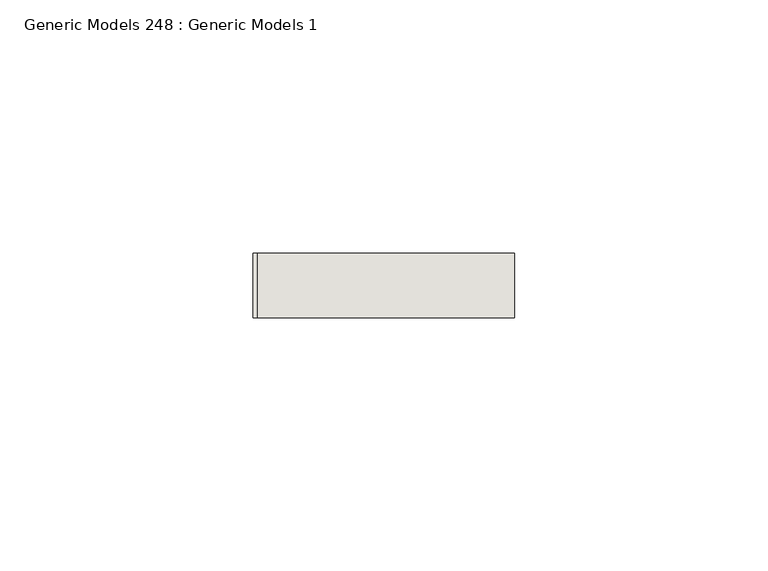
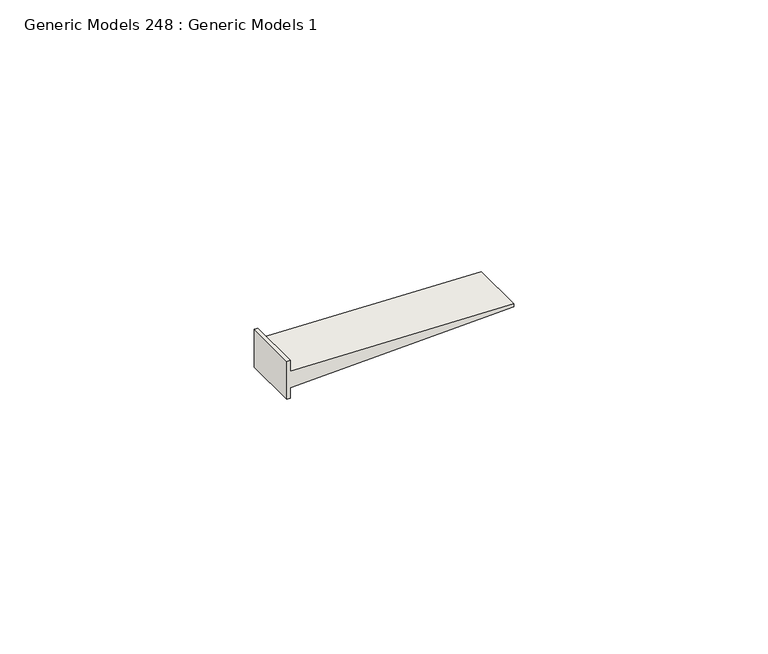
"""IFC4 building model written with IfcOpenShell, lengths in millimetres: wall geometry, Generic Models 248 : Generic Models 1."""

import ifcopenshell
import ifcopenshell.guid

model = None  # the IFC model being written
_history = None  # IfcOwnerHistory: only IFC2X3 demands one
_inside = {}  # id of a spatial element -> (the spatial element, [elements in it])
_under = {}  # id of a project, library or spatial element -> (it, [spatial elements below it])
_declared = {}  # id of a project -> (the project, [libraries it declares])
_typed = {}  # id of a type object -> (the type object, [elements of that type])
_made_of = {}  # id of a material, layer set ... -> (it, [elements and type objects made of it])


def new_model(schema):
    """Start an empty IFC model of exactly this schema.

    Asked for "IFC4X3", IfcOpenShell would pick the latest addendum, in which some entities
    have other attributes; the version numbers below select the first issue.
    IFC2X3 requires an IfcOwnerHistory on every rooted entity: one is made here for all.
    """
    global model, _history
    if schema == "IFC4X3":
        model = ifcopenshell.file(schema_version=(4, 3, 0, 0))
    else:
        model = ifcopenshell.file(schema=schema)
    _inside.clear()
    _under.clear()
    _declared.clear()
    _typed.clear()
    _made_of.clear()
    _history = None
    if model.schema == "IFC2X3":
        org = make("IfcOrganization", Name="unknown")
        user = make(
            "IfcPersonAndOrganization",
            ThePerson=make("IfcPerson", FamilyName="unknown"),
            TheOrganization=org,
        )
        app = make(
            "IfcApplication",
            ApplicationDeveloper=org,
            Version="unknown",
            ApplicationFullName="unknown",
            ApplicationIdentifier="unknown",
        )
        _history = make(
            "IfcOwnerHistory",
            OwningUser=user,
            OwningApplication=app,
            ChangeAction="ADDED",
            CreationDate=0,
        )
    return model


def make(cls, **values):
    """One entity of the class cls with the attributes given. An attribute that is None is left unset."""
    return model.create_entity(
        cls, **{name: value for name, value in values.items() if value is not None}
    )


def rooted(cls, **values):
    """An entity with a GlobalId (a new one), such as an element, a storey or a relation."""
    return make(cls, GlobalId=ifcopenshell.guid.new(), OwnerHistory=_history, **values)


def si_unit(unit_type, name, prefix=None):
    """IfcSIUnit, for example si_unit("LENGTHUNIT", "METRE", prefix="MILLI")."""
    return make("IfcSIUnit", UnitType=unit_type, Prefix=prefix, Name=name)


def assignment(units):
    """IfcUnitAssignment: the units of a project."""
    return None if units is None else make("IfcUnitAssignment", Units=units)


def point(xyz):
    """IfcCartesianPoint."""
    return None if xyz is None else make("IfcCartesianPoint", Coordinates=xyz)


def direction(xyz):
    """IfcDirection."""
    return None if xyz is None else make("IfcDirection", DirectionRatios=xyz)


def frame(location, z_axis=None, x_axis=None):
    """IfcAxis2Placement3D, a coordinate frame: its origin and axes. An axis left out is left unset."""
    return make(
        "IfcAxis2Placement3D",
        Location=point(location),
        Axis=direction(z_axis),
        RefDirection=direction(x_axis),
    )


def origin():
    """The frame at (0, 0, 0) with its axes left unset."""
    return frame((0.0, 0.0, 0.0))


def place(relative_to, where):
    """IfcLocalPlacement: puts the frame where relative to a parent placement (None: the world)."""
    return make(
        "IfcLocalPlacement", PlacementRelTo=relative_to, RelativePlacement=where
    )


def context(
    kind, dimensions, precision=None, world=None, true_north=None, identifier=None
):
    """IfcGeometricRepresentationContext, for example the 3D "Model" context."""
    return make(
        "IfcGeometricRepresentationContext",
        ContextIdentifier=identifier,
        ContextType=kind,
        CoordinateSpaceDimension=dimensions,
        Precision=precision,
        WorldCoordinateSystem=world,
        TrueNorth=true_north,
    )


def project(units=None, contexts=None):
    """IfcProject with its units and contexts."""
    return rooted(
        "IfcProject",
        Name="project",
        RepresentationContexts=contexts,
        UnitsInContext=assignment(units),
    )


def spatial(cls, under=None, at=None, **own):
    """A site, building, storey or space (cls), placed at a placement, below another one or the project."""
    s = rooted(cls, ObjectPlacement=at, **own)
    if under is not None:
        _under.setdefault(under.id(), (under, []))[1].append(s)
    return s


def polyline(points):
    """IfcPolyline through the points."""
    return make("IfcPolyline", Points=[point(p) for p in points])


def outline(outer, holes=None, kind="AREA"):
    """IfcArbitraryClosedProfileDef: a profile drawn as a closed curve; with holes, ...WithVoids."""
    if holes is None:
        return make("IfcArbitraryClosedProfileDef", ProfileType=kind, OuterCurve=outer)
    return make(
        "IfcArbitraryProfileDefWithVoids",
        ProfileType=kind,
        OuterCurve=outer,
        InnerCurves=holes,
    )


def extrude(swept, where, along, depth):
    """IfcExtrudedAreaSolid: the profile swept, set in the frame where, extruded along a direction by depth."""
    return make(
        "IfcExtrudedAreaSolid",
        SweptArea=swept,
        Position=where,
        ExtrudedDirection=direction(along),
        Depth=depth,
    )


def shape(context_of_items, identifier, shape_type, items):
    """IfcShapeRepresentation: the items that make up one representation, for example the "Body"."""
    return make(
        "IfcShapeRepresentation",
        ContextOfItems=context_of_items,
        RepresentationIdentifier=identifier,
        RepresentationType=shape_type,
        Items=items,
    )


def source(mapping_origin, context_of_items, identifier, shape_type, items):
    """IfcRepresentationMap: a shape defined once, which mapped items show again and again."""
    return make(
        "IfcRepresentationMap",
        MappingOrigin=mapping_origin,
        MappedRepresentation=shape(context_of_items, identifier, shape_type, items),
    )


def transform(
    local_origin,
    x_axis=None,
    y_axis=None,
    z_axis=None,
    scale=None,
    scale2=None,
    scale3=None,
    uniform=True,
):
    """IfcCartesianTransformationOperator3D, or its non-uniform kind. x_axis, y_axis, z_axis: its Axis1, 2, 3."""
    if uniform:
        return make(
            "IfcCartesianTransformationOperator3D",
            Axis1=direction(x_axis),
            Axis2=direction(y_axis),
            LocalOrigin=point(local_origin),
            Scale=scale,
            Axis3=direction(z_axis),
        )
    return make(
        "IfcCartesianTransformationOperator3DnonUniform",
        Axis1=direction(x_axis),
        Axis2=direction(y_axis),
        LocalOrigin=point(local_origin),
        Scale=scale,
        Axis3=direction(z_axis),
        Scale2=scale2,
        Scale3=scale3,
    )


def mapped(mapping_source, mapping_target):
    """IfcMappedItem: shows the shape of a source again, moved by a transform."""
    return make(
        "IfcMappedItem", MappingSource=mapping_source, MappingTarget=mapping_target
    )


def made_of(thing, what):
    """Note that an element or type object is made of a material, layer set ...; save() writes the relation."""
    if what is not None:
        _made_of.setdefault(what.id(), (what, []))[1].append(thing)
    return thing


def element(
    cls,
    number,
    at=None,
    inside=None,
    cuts=None,
    type_object=None,
    material=None,
    context=None,
    identifier="Body",
    shape_type=None,
    held_by="IfcProductDefinitionShape",
    body=None,
    shapes=None,
    **own,
):
    """One element of the class cls, such as IfcWall. Its Tag is "e" and its number.

    at: its placement. inside: the storey or other place that contains it. cuts: it is an
    opening in that element (IfcRelVoidsElement). A single representation is given by context,
    identifier, shape_type and body (its items); several are given by shapes. held_by: the class
    of the entity that holds the representations. save() writes the other relations.
    """
    e = rooted(cls, Tag="e%d" % number, ObjectPlacement=at, **own)
    if body is not None:
        shapes = [shape(context, identifier, shape_type, body)]
    if shapes is not None:
        e.Representation = make(held_by, Representations=shapes)
    if inside is not None:
        _inside.setdefault(inside.id(), (inside, []))[1].append(e)
    if cuts is not None:
        rooted(
            "IfcRelVoidsElement", RelatingBuildingElement=cuts, RelatedOpeningElement=e
        )
    if type_object is not None:
        _typed.setdefault(type_object.id(), (type_object, []))[1].append(e)
    return made_of(e, material)


def aggregate(whole, parts):
    """IfcRelAggregates: a whole, such as a stair, and the parts it consists of."""
    return rooted("IfcRelAggregates", RelatingObject=whole, RelatedObjects=parts)


def save(model, path):
    """Write the relations noted so far, then the file.

    IfcRelAggregates (storeys below a building ...), IfcRelContainedInSpatialStructure (elements
    in a storey), IfcRelDefinesByType, IfcRelAssociatesMaterial and IfcRelDeclares: one each for
    every whole, place, type object, material and project.
    """
    for whole, parts in _under.values():
        aggregate(whole, parts)
    for where, things in _inside.values():
        rooted(
            "IfcRelContainedInSpatialStructure",
            RelatedElements=things,
            RelatingStructure=where,
        )
    for kind, things in _typed.values():
        rooted("IfcRelDefinesByType", RelatedObjects=things, RelatingType=kind)
    for what, things in _made_of.values():
        rooted("IfcRelAssociatesMaterial", RelatedObjects=things, RelatingMaterial=what)
    for by, libraries in _declared.values():
        rooted("IfcRelDeclares", RelatingContext=by, RelatedDefinitions=libraries)
    model.write(path)


def generic_models_248_generic_models_1_07be3612(model_context):
    return source(origin(), model_context, "Body", "SweptSolid", [
        extrude(outline(polyline([(5490.9466, 49678.43125), (5481.8534, 49678.43125), (5481.8534, 49679.225), (5484.4032636, 49679.225), (5486.0006527, 49730.025), (5486.7993473, 49730.025), (5488.3967364, 49679.225), (5490.9466, 49679.225), (5490.9466, 49678.43125)])), frame((0.0, 565.15, 0.0), z_axis=(0.0, 1.0, 0.0), x_axis=(0.0, 0.0, 1.0)), (0.0, 0.0, 1.0), 12.7),
    ])


if __name__ == "__main__":
    model = new_model("IFC4")
    model_context = context("Model", 3, world=origin())
    ifc_project = project(units=[si_unit("LENGTHUNIT", "METRE", prefix="MILLI")], contexts=[model_context])
    site = spatial("IfcSite", under=ifc_project)
    building = spatial("IfcBuilding", under=site)
    placement = place(None, origin())
    generic_models_248_generic_models_1_shape = generic_models_248_generic_models_1_07be3612(model_context)
    element("IfcWall", 1, ObjectType="Generic Models 248 : Generic Models 1", at=placement, inside=building, context=model_context, shape_type="MappedRepresentation", body=[
        mapped(generic_models_248_generic_models_1_shape, transform((0.0, 0.0, 0.0), x_axis=(1.0, 0.0, 0.0), y_axis=(0.0, 1.0, 0.0), z_axis=(0.0, 0.0, 1.0))),
    ])
    save(model, "model.ifc")

# Revit data of these elements
# Element 1 (IfcWall, "Generic Models 248 : Generic Models 1")
#   Materials on its faces: "ATTACH GYPSUM BOARD TO STUDS AND NOT TO TOP TRACK"
# Materials
#   "ATTACH GYPSUM BOARD TO STUDS AND NOT TO TOP TRACK": class "Generic", colour RGB 48 48 48, transparency 0, Cost = 0
